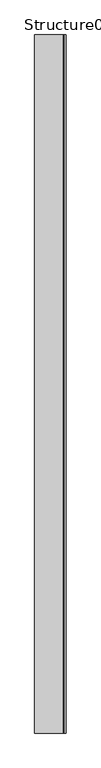
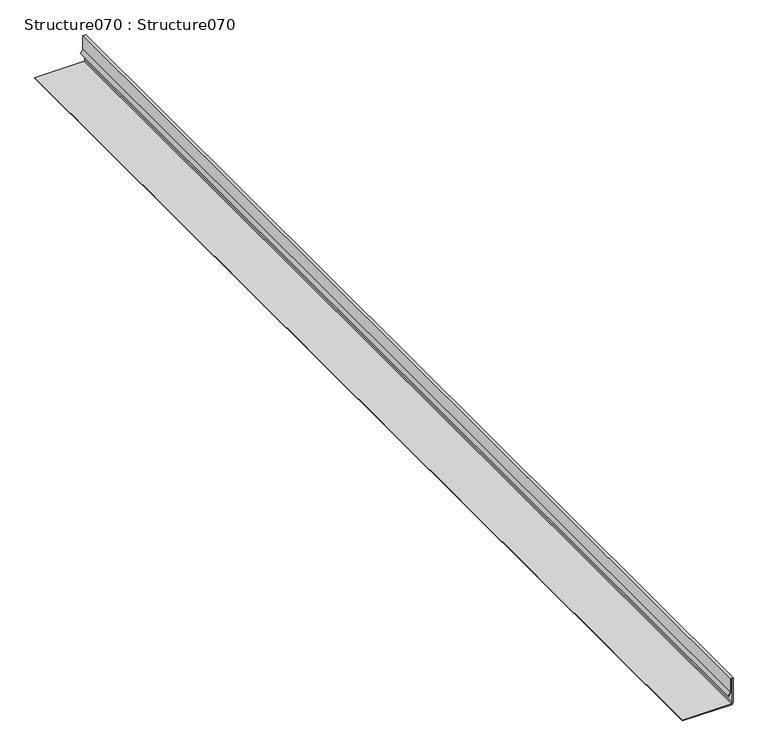
"""IFC4 building model written with IfcOpenShell, lengths in millimetres: proxy geometry, Structure070 : Structure070."""

from ifc_helpers import new_model, si_unit, frame, origin, place, context, project, spatial, polyline, outline, extrude, source, transform, mapped, element, save


def structure070_structure070_b5277a4f(model_context):
    return source(origin(), model_context, "Body", "SweptSolid", [
        extrude(outline(polyline([(42584.5106533, 5852.9658986), (42584.5106533, 5765.1118921), (42583.3200283, 5765.1118921), (42583.3200283, 5853.4590716), (42585.4156482, 5855.5546915), (42633.2240899, 5855.5546915), (42633.2240899, 5850.2372889), (42607.754677, 5850.2372889), (42600.8896725, 5847.1183441), (42600.3864926, 5848.1974168), (42607.0333911, 5851.2969164), (42632.0334649, 5851.4279139), (42632.0334649, 5854.3640665), (42585.9088212, 5854.3640665), (42584.5106533, 5852.9658986)])), frame((0.0, -1052.8906574, 0.0), z_axis=(0.0, 1.0, 0.0), x_axis=(0.0, 0.0, 1.0)), (0.0, 0.0, 1.0), 1999.85),
    ])


if __name__ == "__main__":
    model = new_model("IFC4")
    model_context = context("Model", 3, world=origin())
    ifc_project = project(units=[si_unit("LENGTHUNIT", "METRE", prefix="MILLI")], contexts=[model_context])
    site = spatial("IfcSite", under=ifc_project)
    building = spatial("IfcBuilding", under=site)
    placement = place(None, origin())
    structure070_structure070_shape = structure070_structure070_b5277a4f(model_context)
    element("IfcBuildingElementProxy", 1, Name="Structure070 : Structure070", ObjectType="Structure070 : Structure070", at=placement, inside=building, context=model_context, shape_type="MappedRepresentation", body=[
        mapped(structure070_structure070_shape, transform((0.0, 0.0, 0.0), x_axis=(1.0, 0.0, 0.0), y_axis=(0.0, 1.0, 0.0), z_axis=(0.0, 0.0, 1.0))),
    ])
    save(model, "model.ifc")

# Revit data of these elements
# Type "Structure070 : Structure070"
#   NameOverride = "Structure070"
# Element 1 (IfcBuildingElementProxy, "Structure070 : Structure070")
#   Materials on its faces: "STANDING SEAM METAL ROOF FOLLOW MANU. RECOMMENDED EDGE/TRANSITION DETAILS"
# Materials
#   "STANDING SEAM METAL ROOF FOLLOW MANU. RECOMMENDED EDGE/TRANSITION DETAILS": class "Unassigned", colour RGB 128 128 128, transparency 0, Cost = 0
